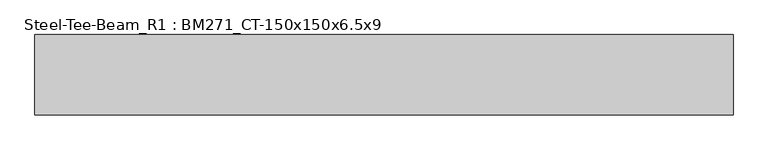
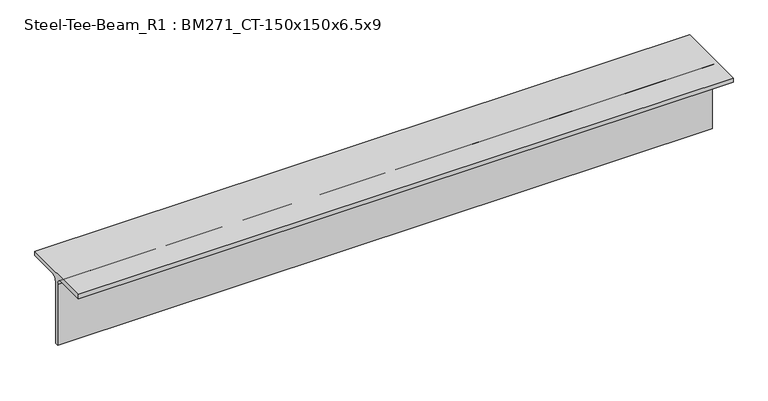
"""IFC4 building model written with IfcOpenShell, lengths in millimetres: member geometry, Steel-Tee-Beam_R1 : BM271_CT-150x150x6.5x9."""

from ifc_helpers import new_model, si_unit, point, frame, frame_2d, origin, place, context, project, spatial, polyline, circle_curve, trimmed, segment, composite_curve, outline, extrude, source, transform, mapped, element, save


def steel_tee_beam_r1_bm271_ct_150x150x6_5x9_46e114fe(model_context):
    return source(origin(), model_context, "Body", "SweptSolid", [
        extrude(outline(composite_curve([segment(polyline([(-75.0, 75.0), (75.0, 75.0), (75.0, 66.0), (16.25, 66.0)]), True, "CONTINUOUS"), segment(trimmed(circle_curve(frame_2d((16.25, 53.0)), 13.0), [point((16.25, 66.0))], [point((3.25, 53.0))], True, "CARTESIAN"), True, "CONTINUOUS"), segment(polyline([(3.25, 53.0), (3.25, -75.0), (-3.25, -75.0), (-3.25, 53.0)]), True, "CONTINUOUS"), segment(trimmed(circle_curve(frame_2d((-16.25, 53.0)), 13.0), [point((-3.25, 53.0))], [point((-16.25, 66.0))], True, "CARTESIAN"), True, "CONTINUOUS"), segment(polyline([(-16.25, 66.0), (-75.0, 66.0), (-75.0, 75.0)]), True, "CONTINUOUS")], self_intersect=False)), frame((-701.7933274, 0.0, 0.0), z_axis=(1.0, 0.0, 0.0), x_axis=(0.0, 1.0, 0.0)), (0.0, 0.0, 1.0), 1302.3874872),
    ])


if __name__ == "__main__":
    model = new_model("IFC4")
    model_context = context("Model", 3, world=origin())
    ifc_project = project(units=[si_unit("LENGTHUNIT", "METRE", prefix="MILLI")], contexts=[model_context])
    site = spatial("IfcSite", under=ifc_project)
    building = spatial("IfcBuilding", under=site)
    placement = place(None, origin())
    steel_tee_beam_r1_bm271_ct_150x150x6_5x9_shape = steel_tee_beam_r1_bm271_ct_150x150x6_5x9_46e114fe(model_context)
    element("IfcMember", 1, ObjectType="Steel-Tee-Beam_R1 : BM271_CT-150x150x6.5x9", at=placement, inside=building, context=model_context, shape_type="MappedRepresentation", body=[
        mapped(steel_tee_beam_r1_bm271_ct_150x150x6_5x9_shape, transform((0.0, 0.0, 0.0), x_axis=(1.0, 0.0, 0.0), y_axis=(0.0, 1.0, 0.0), z_axis=(0.0, 0.0, 1.0))),
    ])
    save(model, "model.ifc")

# Revit data of these elements
# Type "Steel-Tee-Beam_R1 : BM271_CT-150x150x6.5x9"
#   Keynote = "CT-150x150x6.5x9"
#   Surface Area = 0.588841 m²/m
#   Section Area = 23.3904 cm²
#   Mass per Unit Length = 18.3614 kg/m
#   Length [instance default] = 1.5240 m
#   bf = 0.1500 m
#   d = 0.1500 m
#   k = 0.0220 m
#   r = 0.0130 m
#   tf = 0.0090 m
#   tw = 0.0065 m
#   hec_material4 [instance default] = none
#   hec_material3 [instance default] = none
#   hec_material2 [instance default] = none
#   hec_material1 [instance default] = none
#   Structural Material [instance default] = Steel, 45-345
#   Assembly Code = ""
# Element 1 (IfcMember, "Steel-Tee-Beam_R1 : BM271_CT-150x150x6.5x9")
#   Structural Material = none
# Materials
#   "Steel, 45-345": class "Metal", colour RGB 189 187 185, transparency 0, Description = "Steel 345 MPa", Cost = 0
